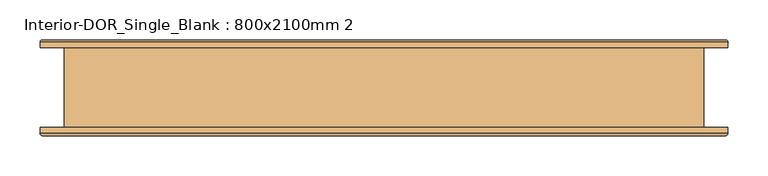
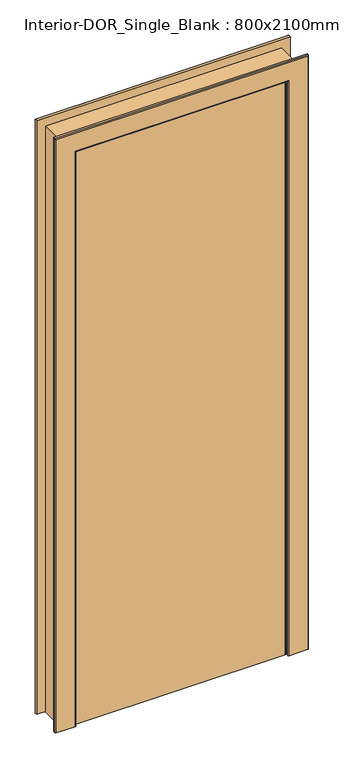
"""IFC4 building model written with IfcOpenShell, lengths in millimetres: door geometry, Interior-DOR_Single_Blank : 800x2100mm 2."""

from ifc_helpers import new_model, si_unit, frame, origin, origin_with_axes, place, context, project, spatial, polyline, circle_curve, ellipse_curve, outline, extrude, faceted_brep, source, transform, mapped, element, save
from ifc_brep_helpers import plane_surface, cylinder_surface, advanced_brep


def interior_dor_single_blank_800x2100mm_2_84615f2d(model_context):
    return source(origin(), model_context, "Body", "SolidModel", [
        advanced_brep(
        [(-360.0, -50.0, 0.0), (-360.0, -57.0, 0.0), (-363.0, -60.0, 0.0), (-427.0, -60.0, 0.0), (-430.0, -57.0, 0.0), (-430.0, -50.0, 0.0), (-360.0, -50.0, 2060.0), (-360.0, -57.0, 2060.0), (-363.0, -60.0, 2063.0), (363.0, -60.0, 2063.0), (363.0, -60.0, 0.0), (427.0, -60.0, 0.0), (427.0, -60.0, 2127.0), (-427.0, -60.0, 2127.0), (-430.0, -57.0, 2130.0), (-430.0, -50.0, 2130.0), (430.0, -50.0, 2130.0), (430.0, -50.0, 0.0), (360.0, -50.0, 0.0), (360.0, -50.0, 2060.0), (360.0, -57.0, 2060.0), (360.0, -57.0, 0.0), (430.0, -57.0, 0.0), (430.0, -57.0, 2130.0)],
        [
            (0, 1),
            (1, 2, circle_curve(frame((-363.0, -57.0, 0.0), z_axis=(0.0, 0.0, -1.0), x_axis=(-1.0, 0.0, 0.0)), 3.0)),
            (2, 3),
            (3, 4, circle_curve(frame((-427.0, -57.0, 0.0), z_axis=(0.0, 0.0, -1.0), x_axis=(-1.0, 0.0, 0.0)), 3.0)),
            (4, 5),
            (5, 0),
            (0, 6),
            (6, 7),
            (7, 1),
            (7, 8, ellipse_curve(frame((-363.0, -57.0, 2063.0), z_axis=(-0.7071067811865475, 0.0, -0.7071067811865475), x_axis=(0.7071067811865474, 0.0, -0.7071067811865476)), 4.2426407, 3.0)),
            (8, 2),
            (8, 9),
            (9, 10),
            (10, 11),
            (11, 12),
            (12, 13),
            (13, 3),
            (13, 14, ellipse_curve(frame((-427.0, -57.0, 2127.0), z_axis=(-0.7071067811865475, 0.0, -0.7071067811865475), x_axis=(0.7071067811865474, 0.0, -0.7071067811865476)), 4.2426407, 3.0)),
            (14, 4),
            (14, 15),
            (15, 5),
            (15, 16),
            (16, 17),
            (17, 18),
            (18, 19),
            (19, 6),
            (9, 20, ellipse_curve(frame((363.0, -57.0, 2063.0), z_axis=(0.7071067811865475, 0.0, -0.7071067811865475), x_axis=(0.7071067811865474, 0.0, 0.7071067811865476)), 4.2426407, 3.0)),
            (20, 21),
            (21, 10, circle_curve(frame((363.0, -57.0, 0.0), z_axis=(0.0, 0.0, 1.0), x_axis=(1.0, 0.0, 0.0)), 3.0)),
            (17, 22),
            (22, 11, circle_curve(frame((427.0, -57.0, 0.0), z_axis=(0.0, 0.0, -1.0), x_axis=(1.0, 0.0, 0.0)), 3.0)),
            (21, 18),
            (23, 12, ellipse_curve(frame((427.0, -57.0, 2127.0), z_axis=(0.7071067811865475, 0.0, -0.7071067811865475), x_axis=(0.7071067811865474, 0.0, 0.7071067811865476)), 4.2426407, 3.0)),
            (22, 23),
            (16, 23),
            (20, 19),
            (20, 7),
            (23, 14),
        ],
        [
            plane_surface(frame((-400.0, 50.0, 0.0), z_axis=(0.0, 0.0, -1.0), x_axis=(0.0, -1.0, 0.0))),
            plane_surface(frame((-360.0, -50.0, 0.0), z_axis=(1.0, 0.0, 0.0), x_axis=(0.0, 0.0, 1.0))),
            cylinder_surface(frame((-363.0, -57.0, 0.0), z_axis=(0.0, 0.0, -1.0), x_axis=(-1.0, 0.0, 0.0)), 3.0),
            plane_surface(frame((-363.0, -60.0, 0.0), z_axis=(0.0, -1.0, 0.0), x_axis=(0.0, 0.0, 1.0))),
            cylinder_surface(frame((-427.0, -57.0, 0.0), z_axis=(0.0, 0.0, -1.0), x_axis=(-1.0, 0.0, 0.0)), 3.0),
            plane_surface(frame((-430.0, -57.0, 0.0), z_axis=(-1.0, 0.0, 0.0), x_axis=(0.0, 0.0, 1.0))),
            plane_surface(frame((-430.0, -50.0, 0.0), z_axis=(0.0, 1.0, 0.0), x_axis=(0.0, 0.0, 1.0))),
            cylinder_surface(frame((363.0, -57.0, 2100.0), z_axis=(0.0, 0.0, 1.0), x_axis=(1.0, 0.0, 0.0)), 3.0),
            plane_surface(frame((400.0, 50.0, 0.0), z_axis=(0.0, 0.0, -1.0), x_axis=(0.0, -1.0, 0.0))),
            cylinder_surface(frame((427.0, -57.0, 2100.0), z_axis=(0.0, 0.0, 1.0), x_axis=(1.0, 0.0, 0.0)), 3.0),
            plane_surface(frame((430.0, -57.0, 2130.0), z_axis=(1.0, 0.0, 0.0), x_axis=(0.0, 0.0, -1.0))),
            plane_surface(frame((360.0, -50.0, 2060.0), z_axis=(-1.0, 0.0, 0.0), x_axis=(0.0, 0.0, -1.0))),
            plane_surface(frame((-360.0, -50.0, 2060.0), z_axis=(0.0, 0.0, -1.0), x_axis=(1.0, 0.0, 0.0))),
            cylinder_surface(frame((-400.0, -57.0, 2063.0), z_axis=(-1.0, 0.0, 0.0), x_axis=(0.0, 0.0, 1.0)), 3.0),
            cylinder_surface(frame((-400.0, -57.0, 2127.0), z_axis=(-1.0, 0.0, 0.0), x_axis=(0.0, 0.0, 1.0)), 3.0),
            plane_surface(frame((-430.0, -57.0, 2130.0), z_axis=(0.0, 0.0, 1.0), x_axis=(1.0, 0.0, 0.0))),
        ],
        [
            (0, [[1, 2, 3, 4, 5, 6]]),
            (1, [[-1, 7, 8, 9]]),
            (2, [[-2, -9, 10, 11]]),
            (3, [[-3, -11, 12, 13, 14, 15, 16, 17]]),
            (4, [[-4, -17, 18, 19]]),
            (5, [[-5, -19, 20, 21]]),
            (6, [[-6, -21, 22, 23, 24, 25, 26, -7]]),
            (7, [[27, 28, 29, -13]]),
            (8, [[-24, 30, 31, -14, -29, 32]]),
            (9, [[33, -15, -31, 34]]),
            (10, [[35, -34, -30, -23]]),
            (11, [[36, -25, -32, -28]]),
            (12, [[-8, -26, -36, 37]]),
            (13, [[-10, -37, -27, -12]]),
            (14, [[-18, -16, -33, 38]]),
            (15, [[-20, -38, -35, -22]]),
        ],
    ),
        advanced_brep(
        [(-430.0, 50.0, 0.0), (-430.0, 57.0, 0.0), (-427.0, 60.0, 0.0), (-363.0, 60.0, 0.0), (-360.0, 57.0, 0.0), (-360.0, 50.0, 0.0), (-430.0, 50.0, 2130.0), (-430.0, 57.0, 2130.0), (-427.0, 60.0, 2127.0), (427.0, 60.0, 2127.0), (427.0, 60.0, 0.0), (363.0, 60.0, 0.0), (363.0, 60.0, 2063.0), (-363.0, 60.0, 2063.0), (-360.0, 57.0, 2060.0), (-360.0, 50.0, 2060.0), (360.0, 50.0, 2060.0), (360.0, 50.0, 0.0), (430.0, 50.0, 0.0), (430.0, 50.0, 2130.0), (430.0, 57.0, 2130.0), (430.0, 57.0, 0.0), (360.0, 57.0, 0.0), (360.0, 57.0, 2060.0)],
        [
            (0, 1),
            (1, 2, circle_curve(frame((-427.0, 57.0, 0.0), z_axis=(0.0, 0.0, -1.0), x_axis=(-1.0, 0.0, 0.0)), 3.0)),
            (2, 3),
            (3, 4, circle_curve(frame((-363.0, 57.0, 0.0), z_axis=(0.0, 0.0, -1.0), x_axis=(-1.0, 0.0, 0.0)), 3.0)),
            (4, 5),
            (5, 0),
            (0, 6),
            (6, 7),
            (7, 1),
            (7, 8, ellipse_curve(frame((-427.0, 57.0, 2127.0), z_axis=(-0.7071067811865475, 0.0, -0.7071067811865475), x_axis=(0.7071067811865474, 0.0, -0.7071067811865476)), 4.2426407, 3.0)),
            (8, 2),
            (8, 9),
            (9, 10),
            (10, 11),
            (11, 12),
            (12, 13),
            (13, 3),
            (13, 14, ellipse_curve(frame((-363.0, 57.0, 2063.0), z_axis=(-0.7071067811865475, 0.0, -0.7071067811865475), x_axis=(0.7071067811865474, 0.0, -0.7071067811865476)), 4.2426407, 3.0)),
            (14, 4),
            (14, 15),
            (15, 5),
            (15, 16),
            (16, 17),
            (17, 18),
            (18, 19),
            (19, 6),
            (9, 20, ellipse_curve(frame((427.0, 57.0, 2127.0), z_axis=(0.7071067811865475, 0.0, -0.7071067811865475), x_axis=(0.7071067811865474, 0.0, 0.7071067811865476)), 4.2426407, 3.0)),
            (20, 21),
            (21, 10, circle_curve(frame((427.0, 57.0, 0.0), z_axis=(0.0, 0.0, 1.0), x_axis=(1.0, 0.0, 0.0)), 3.0)),
            (17, 22),
            (22, 11, circle_curve(frame((363.0, 57.0, 0.0), z_axis=(0.0, 0.0, -1.0), x_axis=(1.0, 0.0, 0.0)), 3.0)),
            (21, 18),
            (23, 12, ellipse_curve(frame((363.0, 57.0, 2063.0), z_axis=(0.7071067811865475, 0.0, -0.7071067811865475), x_axis=(0.7071067811865474, 0.0, 0.7071067811865476)), 4.2426407, 3.0)),
            (22, 23),
            (16, 23),
            (20, 19),
            (20, 7),
            (23, 14),
        ],
        [
            plane_surface(frame((-400.0, 50.0, 0.0), z_axis=(0.0, 0.0, -1.0), x_axis=(0.0, -1.0, 0.0))),
            plane_surface(frame((-430.0, 50.0, 0.0), z_axis=(-1.0, 0.0, 0.0), x_axis=(0.0, 0.0, 1.0))),
            cylinder_surface(frame((-427.0, 57.0, 0.0), z_axis=(0.0, 0.0, -1.0), x_axis=(-1.0, 0.0, 0.0)), 3.0),
            plane_surface(frame((-427.0, 60.0, 0.0), z_axis=(0.0, 1.0, 0.0), x_axis=(0.0, 0.0, 1.0))),
            cylinder_surface(frame((-363.0, 57.0, 0.0), z_axis=(0.0, 0.0, -1.0), x_axis=(-1.0, 0.0, 0.0)), 3.0),
            plane_surface(frame((-360.0, 57.0, 0.0), z_axis=(1.0, 0.0, 0.0), x_axis=(0.0, 0.0, 1.0))),
            plane_surface(frame((-360.0, 50.0, 0.0), z_axis=(0.0, -1.0, 0.0), x_axis=(0.0, 0.0, 1.0))),
            cylinder_surface(frame((427.0, 57.0, 2100.0), z_axis=(0.0, 0.0, 1.0), x_axis=(1.0, 0.0, 0.0)), 3.0),
            plane_surface(frame((400.0, 50.0, 0.0), z_axis=(0.0, 0.0, -1.0), x_axis=(0.0, -1.0, 0.0))),
            cylinder_surface(frame((363.0, 57.0, 2100.0), z_axis=(0.0, 0.0, 1.0), x_axis=(1.0, 0.0, 0.0)), 3.0),
            plane_surface(frame((360.0, 57.0, 2060.0), z_axis=(-1.0, 0.0, 0.0), x_axis=(0.0, 0.0, -1.0))),
            plane_surface(frame((430.0, 50.0, 2130.0), z_axis=(1.0, 0.0, 0.0), x_axis=(0.0, 0.0, -1.0))),
            plane_surface(frame((-430.0, 50.0, 2130.0), z_axis=(0.0, 0.0, 1.0), x_axis=(1.0, 0.0, 0.0))),
            cylinder_surface(frame((-400.0, 57.0, 2127.0), z_axis=(-1.0, 0.0, 0.0), x_axis=(0.0, 0.0, 1.0)), 3.0),
            cylinder_surface(frame((-400.0, 57.0, 2063.0), z_axis=(-1.0, 0.0, 0.0), x_axis=(0.0, 0.0, 1.0)), 3.0),
            plane_surface(frame((-360.0, 57.0, 2060.0), z_axis=(0.0, 0.0, -1.0), x_axis=(1.0, 0.0, 0.0))),
        ],
        [
            (0, [[1, 2, 3, 4, 5, 6]]),
            (1, [[-1, 7, 8, 9]]),
            (2, [[-2, -9, 10, 11]]),
            (3, [[-3, -11, 12, 13, 14, 15, 16, 17]]),
            (4, [[-4, -17, 18, 19]]),
            (5, [[-5, -19, 20, 21]]),
            (6, [[-6, -21, 22, 23, 24, 25, 26, -7]]),
            (7, [[27, 28, 29, -13]]),
            (8, [[-24, 30, 31, -14, -29, 32]]),
            (9, [[33, -15, -31, 34]]),
            (10, [[35, -34, -30, -23]]),
            (11, [[36, -25, -32, -28]]),
            (12, [[-8, -26, -36, 37]]),
            (13, [[-10, -37, -27, -12]]),
            (14, [[-18, -16, -33, 38]]),
            (15, [[-20, -38, -35, -22]]),
        ],
    ),
        faceted_brep([(-400.0, 50.0, 0.0), (-355.0, 50.0, 0.0), (-355.0, 35.0, 0.0), (-335.0, 35.0, 0.0), (-335.0, -5.0, 0.0), (-355.0, -5.0, 0.0), (-355.0, -50.0, 0.0), (-400.0, -50.0, 0.0), (-400.0, 50.0, 2100.0), (400.0, 50.0, 2100.0), (400.0, 50.0, 0.0), (355.0, 50.0, 0.0), (355.0, 50.0, 2055.0), (-355.0, 50.0, 2055.0), (-355.0, 35.0, 2055.0), (355.0, 35.0, 2055.0), (355.0, 35.0, 0.0), (335.0, 35.0, 0.0), (335.0, 35.0, 2035.0), (-335.0, 35.0, 2035.0), (-335.0, -5.0, 2035.0), (335.0, -5.0, 2035.0), (335.0, -5.0, 0.0), (355.0, -5.0, 0.0), (355.0, -5.0, 2055.0), (-355.0, -5.0, 2055.0), (-355.0, -50.0, 2055.0), (355.0, -50.0, 2055.0), (355.0, -50.0, 0.0), (400.0, -50.0, 0.0), (400.0, -50.0, 2100.0), (-400.0, -50.0, 2100.0)], [[[0, 1, 2, 3, 4, 5, 6, 7]], [[1, 0, 8, 9, 10, 11, 12, 13]], [[2, 1, 13, 14]], [[3, 2, 14, 15, 16, 17, 18, 19]], [[4, 3, 19, 20]], [[5, 4, 20, 21, 22, 23, 24, 25]], [[6, 5, 25, 26]], [[7, 6, 26, 27, 28, 29, 30, 31]], [[0, 7, 31, 8]], [[9, 30, 29, 10]], [[10, 29, 28, 23, 22, 17, 16, 11]], [[15, 12, 11, 16]], [[21, 18, 17, 22]], [[27, 24, 23, 28]], [[20, 19, 18, 21]], [[26, 25, 24, 27]], [[8, 31, 30, 9]], [[14, 13, 12, 15]]]),
        extrude(outline(polyline([(355.0, -50.0), (-355.0, -50.0), (-355.0, -5.0), (355.0, -5.0), (355.0, -50.0)])), origin_with_axes(), (0.0, 0.0, 1.0), 2055.0),
    ])


if __name__ == "__main__":
    model = new_model("IFC4")
    model_context = context("Model", 3, world=origin())
    ifc_project = project(units=[si_unit("LENGTHUNIT", "METRE", prefix="MILLI")], contexts=[model_context])
    site = spatial("IfcSite", under=ifc_project)
    building = spatial("IfcBuilding", under=site)
    placement = place(None, origin())
    interior_dor_single_blank_800x2100mm_2_shape = interior_dor_single_blank_800x2100mm_2_84615f2d(model_context)
    element("IfcDoor", 1, ObjectType="Interior-DOR_Single_Blank : 800x2100mm 2", at=placement, inside=building, context=model_context, shape_type="MappedRepresentation", body=[
        mapped(interior_dor_single_blank_800x2100mm_2_shape, transform((0.0, 0.0, 0.0), x_axis=(1.0, 0.0, 0.0), y_axis=(0.0, 1.0, 0.0), z_axis=(0.0, 0.0, 1.0))),
    ])
    save(model, "model.ifc")

# Revit data of these elements
# Type "Interior-DOR_Single_Blank : 800x2100mm 2"
#   Type IfcGUID = "0dwJ1JWsv3L8A_XhzwP5MW"
#   Assembly Code = "C1020120"
#   Type Mark = "195"
#   Classification.Uniclass.EF.Number = "EF_25_30"
#   Classification.Uniclass.EF.Description = "Doors and windows"
#   WindLoadRating = "n/a"
#   WaterTightnessRating = "n/a"
#   WarrantyStartDate [instance default] = "1900-12-31T23:59:59"
#   WarrantyGuarantorParts = "n/a"
#   WarrantyGuarantorLabor = "n/a"
#   WarrantyDurationUnit = "year"
#   WarrantyDurationParts = "n/a"
#   WarrantyDurationLabor = "n/a"
#   WarrantyDescription = "n/a"
#   Version = "2"
#   Uniclass2015Version = "Systems v1.9"
#   Uniclass2015Title = "Doorset systems"
#   Uniclass2015Code = "Ss_25_30_20_25"
#   URL = "www.nationalbimlibrary.com"
#   TagNumber [instance default] = "n/a"
#   SustainabilityPerformance = "n/a"
#   Status = "UNSET"
#   Size = "1010 x 2100 mm"
#   Shape = "n/a"
#   SerialNumber [instance default] = "n/a"
#   SecurityRating = "n/a"
#   Revision = "n/a"
#   ReplacementCost = "n/a"
#   Reference = "n/a"
#   ProductInformation = "n/a"
#   Operation = "SINGLE_SWING_RIGHT"
#   OmniClassVersion = "Table 22 2012-05-16"
#   OmniClassTitle = "Doors and Frames"
#   OmniClassCode = "22-08 10 00"
#   Name = "DoorsetSystem_Interior-Single_Blank"
#   NBSReference = "25-50-20/120"
#   NBSDescription = "Doorset system"
#   NBSCertification = "www.nationalbimlibrary.com/cert/mlf45nxc"
#   ModelReference = "Interior Single Door"
#   ModelNumber = "n/a"
#   Model = "Interior Single Door"
#   MechanicalLoadRating = "n/a"
#   Material = "n/a"
#   ManufacturerURL = "n/a"
#   ManufacturerName = "n/a"
#   Manufacturer = "info@theNBS.com"
#   InstallationDate [instance default] = "1900-12-31T23:59:59"
#   IfcExportType = "DOOR"
#   IfcExportAs = "IfcDoorType"
#   HygrothermalRating = "n/a"
#   Grade = "n/a"
#   FireRating = "n/a"
#   Fire Rating = "n/a"
#   Finish = "n/a"
#   Features = "n/a"
#   ExpectedLife = "n/a"
#   DurationUnit = "n/a"
#   DurabilityRating = "n/a"
#   DoorNumber [instance default] = "n/a"
#   Description = "Generic single interior door"
#   Construction Type = "USERDEFINED"
#   Constituents = "n/a"
#   ComponentNumber [instance default] = "n/a"
#   Color = "n/a"
#   CodePerformance = "n/a"
#   Category = "Ss_25_30_20_25:Doorset systems"
#   BarCode [instance default] = "n/a"
#   BIMObjectName = "NBS_DoorsetSystem_Interior-Single_Blank"
#   Author = "NBS"
#   AssetType = "Fixed"
#   AssetIdentifier [instance default] = "n/a"
#   AcousticRating = "n/a"
#   AccessibilityPerformance = "n/a"
#   Width = 0.8 m
#   WallThickness [instance default] = 0.15 m
#   ThresholdHeight = 0.015 m
#   Thickness = 0.15 m
#   ThermalTransmittance = 0
#   StructuralToleranceJamb = 0 m
#   StructuralToleranceHead = 0 m
#   StructuralOpeningWidth = 0.8 m
#   StructuralOpeningHeight = 2.1 m
#   StopProjection = 0.02 m
#   StopDepth = 0.04 m
#   Rough Width [instance default] = 0.8 m
#   Rough Height [instance default] = 2.1 m
#   RebateDepth = 0.045 m
#   PanelWidth = 0.71 m
#   PanelUndercut = 0 m
#   PanelHeight = 2.055 m
#   PanelDepth = 0.045 m
#   OpeningTolerance = 0 m
#   NominalWidth = 0.8 m
#   NominalLength = 0 m
#   NominalHeight = 2.1 m
#   Infiltration = 0
#   Height = 2.1 m
#   GlazingAreaFraction = 0
#   FrameThickness = 0.045 m
#   FrameSetback [instance default] = 0 m
#   FrameDepth [instance default] = 0.15 m
#   FinishThicknessInternal [instance default] = 0 m
#   FinishThicknessExternal [instance default] = 0 m
#   ClearOpeningWidth = 0.67 m
#   ClearOpeningHeight = 2.035 m
#   CalculatedInteriorVoidDepth [instance default] = 0.3 m
#   ArchitraveWidth = 0.07 m
#   ArchitraveThickness = 0.01 m
#   ArchitraveSetbackFromFrameFace = 0.005 m
#   SmokeStop = no
#   SingleRebate = no
#   SelfClosing = no
#   PlantedStop = yes
#   IsExternal = no
#   HasDrive = no
#   HandicapAccessible = no
#   Wall Closure = 4
#   FireExit = no
#   ArchitraveFrontRequired [instance default] = yes
#   ArchitraveBackRequired [instance default] = yes
#   PanelMaterial = NBS_Concept
#   HardwareFinish = NBS_Concept
#   FrameSectionMaterial = NBS_Concept
#   Function = (empty or 0)
#   Cost = 0
# Element 1 (IfcDoor, "Interior-DOR_Single_Blank : 800x2100mm 2")
#   WallThickness = 0.1 m
#   FrameDepth = 0.1 m
#   Materials on its faces: "NBS_Concept"
# Materials
#   "NBS_Concept": class "Generic", colour RGB 255 255 255, transparency 0, Description = "To be specified", Cost = 0
